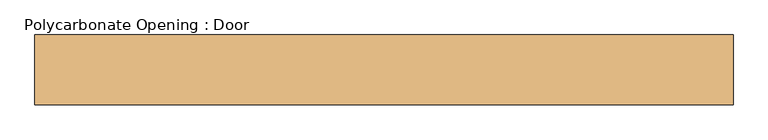
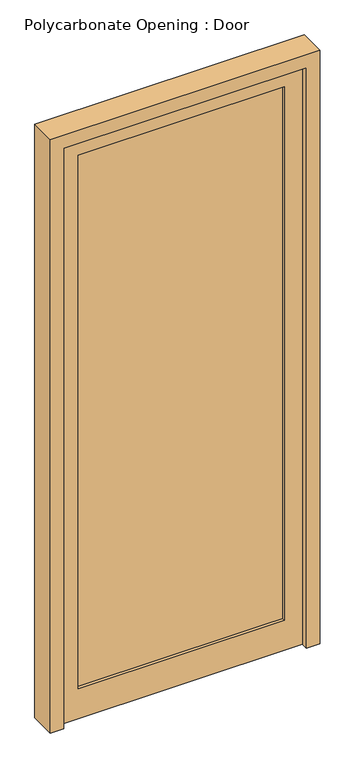
"""IFC4 building model written with IfcOpenShell, lengths in millimetres: door geometry, Polycarbonate Opening : Door."""

from ifc_helpers import new_model, si_unit, frame, origin, place, context, project, spatial, polyline, outline, extrude, source, transform, mapped, element, save


def polycarbonate_opening_door_70b8412c(model_context):
    return source(origin(), model_context, "Body", "SweptSolid", [
        extrude(outline(polyline([(457.2, 0.0), (457.2, -25.4), (-457.2, -25.4), (-457.2, 0.0), (457.2, 0.0)])), frame((0.0, 0.0, 50.8), z_axis=(0.0, 0.0, 1.0), x_axis=(1.0, 0.0, 0.0)), (0.0, 0.0, 1.0), 2260.6),
        extrude(outline(polyline([(2311.4, -457.2), (0.0, -457.2), (0.0, 457.2), (2311.4, 457.2), (2311.4, -457.2)]), holes=[polyline([(119.0625, 388.9375), (119.0625, -388.9375), (2243.1375, -388.9375), (2243.1375, 388.9375), (119.0625, 388.9375)])]), frame((0.0, -38.1, 0.0), z_axis=(0.0, 1.0, 0.0), x_axis=(0.0, 0.0, 1.0)), (0.0, 0.0, 1.0), 50.8),
        extrude(outline(polyline([(2362.2, 508.0), (2362.2, -508.0), (0.0, -508.0), (0.0, -457.2), (2311.4, -457.2), (2311.4, 457.2), (0.0, 457.2), (0.0, 508.0), (2362.2, 508.0)])), frame((0.0, -63.5, 0.0), z_axis=(0.0, 1.0, 0.0), x_axis=(0.0, 0.0, 1.0)), (0.0, 0.0, 1.0), 101.6),
    ])


if __name__ == "__main__":
    model = new_model("IFC4")
    model_context = context("Model", 3, world=origin())
    ifc_project = project(units=[si_unit("LENGTHUNIT", "METRE", prefix="MILLI")], contexts=[model_context])
    site = spatial("IfcSite", under=ifc_project)
    building = spatial("IfcBuilding", under=site)
    placement = place(None, origin())
    polycarbonate_opening_door_shape = polycarbonate_opening_door_70b8412c(model_context)
    element("IfcDoor", 1, ObjectType="Polycarbonate Opening : Door", at=placement, inside=building, context=model_context, shape_type="MappedRepresentation", body=[
        mapped(polycarbonate_opening_door_shape, transform((0.0, 0.0, 0.0), x_axis=(1.0, 0.0, 0.0), y_axis=(0.0, 1.0, 0.0), z_axis=(0.0, 0.0, 1.0))),
    ])
    save(model, "model.ifc")

# Revit data of these elements
# Type "Polycarbonate Opening : Door"
#   Type Mark = "60"
#   OD_DS_Door_Material = "ALUM./GLAZING"
#   OD_DS_Door_Type = "STOREFRONT (NARROW STILE)"
#   OD_DS_Lockset = "ENTRY LOCK (INSIDE ADA LEVER ALWAYS ACTIVE)"
#   Analytic Construction = "<None>"
#   offset [instance default] = 0' - 0 1/2"
#   Stile = 0' - 2 11/16"
#   Mullion Width = 0' - 2"
#   Mullion Depth = 0' - 4"
#   Opening Size [instance default] = 5' - 1.50212"
#   Door Width [instance default] = 5' - 1.50212"
#   Window ON/OFF = yes
#   Door On/Off = no
#   Mullion Material = KAWNEER 260 INSULCLADTM THERMAL ENTRANCE - CLEAR ANODIZED ALUM.
#   Glass Material = TEMPERED INSULATED GLAZING (CARDINAL GLASS LoĒ²-240\nOR EQUIVALENT)
#   Door Material = KAWNEER 260 INSULCLADTM THERMAL ENTRANCE - CLEAR ANODIZED ALUM.
# Element 1 (IfcDoor, "Polycarbonate Opening : Door")
#   Materials on its faces: "KAWNEER 260 INSULCLADTM THERMAL ENTRANCE - CLEAR ANODIZED ALUM.", "TEMPERED INSULATED GLAZING (CARDINAL GLASS LoĒ²-240\nOR EQUIVALENT)"
# Materials
#   "KAWNEER 260 INSULCLADTM THERMAL ENTRANCE - CLEAR ANODIZED ALUM.": class "Metal", colour RGB 244 244 244, transparency 0, Description = "Aluminum 6061", Cost = 0
#   "TEMPERED INSULATED GLAZING (CARDINAL GLASS LoĒ²-240\nOR EQUIVALENT)": class "Glass", colour RGB 196 205 210, transparency 0.85, Description = "Soda Lime Glass", Cost = 0
